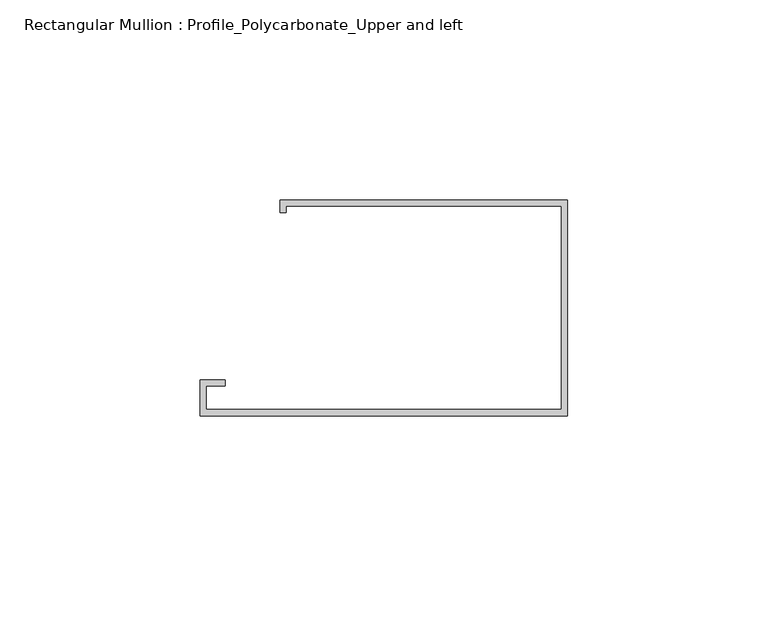
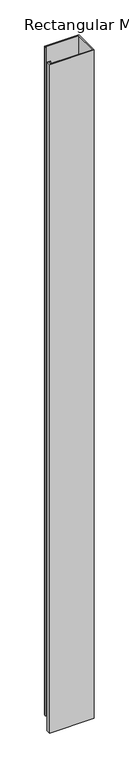
"""IFC4 building model written with IfcOpenShell, lengths in millimetres: member geometry, Rectangular Mullion : Profile_Polycarbonate_Upper and left."""

import ifcopenshell
import ifcopenshell.guid

model = None  # the IFC model being written
_history = None  # IfcOwnerHistory: only IFC2X3 demands one
_inside = {}  # id of a spatial element -> (the spatial element, [elements in it])
_under = {}  # id of a project, library or spatial element -> (it, [spatial elements below it])
_declared = {}  # id of a project -> (the project, [libraries it declares])
_typed = {}  # id of a type object -> (the type object, [elements of that type])
_made_of = {}  # id of a material, layer set ... -> (it, [elements and type objects made of it])


def new_model(schema):
    """Start an empty IFC model of exactly this schema.

    Asked for "IFC4X3", IfcOpenShell would pick the latest addendum, in which some entities
    have other attributes; the version numbers below select the first issue.
    IFC2X3 requires an IfcOwnerHistory on every rooted entity: one is made here for all.
    """
    global model, _history
    if schema == "IFC4X3":
        model = ifcopenshell.file(schema_version=(4, 3, 0, 0))
    else:
        model = ifcopenshell.file(schema=schema)
    _inside.clear()
    _under.clear()
    _declared.clear()
    _typed.clear()
    _made_of.clear()
    _history = None
    if model.schema == "IFC2X3":
        org = make("IfcOrganization", Name="unknown")
        user = make(
            "IfcPersonAndOrganization",
            ThePerson=make("IfcPerson", FamilyName="unknown"),
            TheOrganization=org,
        )
        app = make(
            "IfcApplication",
            ApplicationDeveloper=org,
            Version="unknown",
            ApplicationFullName="unknown",
            ApplicationIdentifier="unknown",
        )
        _history = make(
            "IfcOwnerHistory",
            OwningUser=user,
            OwningApplication=app,
            ChangeAction="ADDED",
            CreationDate=0,
        )
    return model


def make(cls, **values):
    """One entity of the class cls with the attributes given. An attribute that is None is left unset."""
    return model.create_entity(
        cls, **{name: value for name, value in values.items() if value is not None}
    )


def rooted(cls, **values):
    """An entity with a GlobalId (a new one), such as an element, a storey or a relation."""
    return make(cls, GlobalId=ifcopenshell.guid.new(), OwnerHistory=_history, **values)


def si_unit(unit_type, name, prefix=None):
    """IfcSIUnit, for example si_unit("LENGTHUNIT", "METRE", prefix="MILLI")."""
    return make("IfcSIUnit", UnitType=unit_type, Prefix=prefix, Name=name)


def assignment(units):
    """IfcUnitAssignment: the units of a project."""
    return None if units is None else make("IfcUnitAssignment", Units=units)


def point(xyz):
    """IfcCartesianPoint."""
    return None if xyz is None else make("IfcCartesianPoint", Coordinates=xyz)


def direction(xyz):
    """IfcDirection."""
    return None if xyz is None else make("IfcDirection", DirectionRatios=xyz)


def frame(location, z_axis=None, x_axis=None):
    """IfcAxis2Placement3D, a coordinate frame: its origin and axes. An axis left out is left unset."""
    return make(
        "IfcAxis2Placement3D",
        Location=point(location),
        Axis=direction(z_axis),
        RefDirection=direction(x_axis),
    )


def origin():
    """The frame at (0, 0, 0) with its axes left unset."""
    return frame((0.0, 0.0, 0.0))


def place(relative_to, where):
    """IfcLocalPlacement: puts the frame where relative to a parent placement (None: the world)."""
    return make(
        "IfcLocalPlacement", PlacementRelTo=relative_to, RelativePlacement=where
    )


def context(
    kind, dimensions, precision=None, world=None, true_north=None, identifier=None
):
    """IfcGeometricRepresentationContext, for example the 3D "Model" context."""
    return make(
        "IfcGeometricRepresentationContext",
        ContextIdentifier=identifier,
        ContextType=kind,
        CoordinateSpaceDimension=dimensions,
        Precision=precision,
        WorldCoordinateSystem=world,
        TrueNorth=true_north,
    )


def project(units=None, contexts=None):
    """IfcProject with its units and contexts."""
    return rooted(
        "IfcProject",
        Name="project",
        RepresentationContexts=contexts,
        UnitsInContext=assignment(units),
    )


def spatial(cls, under=None, at=None, **own):
    """A site, building, storey or space (cls), placed at a placement, below another one or the project."""
    s = rooted(cls, ObjectPlacement=at, **own)
    if under is not None:
        _under.setdefault(under.id(), (under, []))[1].append(s)
    return s


def polyline(points):
    """IfcPolyline through the points."""
    return make("IfcPolyline", Points=[point(p) for p in points])


def outline(outer, holes=None, kind="AREA"):
    """IfcArbitraryClosedProfileDef: a profile drawn as a closed curve; with holes, ...WithVoids."""
    if holes is None:
        return make("IfcArbitraryClosedProfileDef", ProfileType=kind, OuterCurve=outer)
    return make(
        "IfcArbitraryProfileDefWithVoids",
        ProfileType=kind,
        OuterCurve=outer,
        InnerCurves=holes,
    )


def extrude(swept, where, along, depth):
    """IfcExtrudedAreaSolid: the profile swept, set in the frame where, extruded along a direction by depth."""
    return make(
        "IfcExtrudedAreaSolid",
        SweptArea=swept,
        Position=where,
        ExtrudedDirection=direction(along),
        Depth=depth,
    )


def shape(context_of_items, identifier, shape_type, items):
    """IfcShapeRepresentation: the items that make up one representation, for example the "Body"."""
    return make(
        "IfcShapeRepresentation",
        ContextOfItems=context_of_items,
        RepresentationIdentifier=identifier,
        RepresentationType=shape_type,
        Items=items,
    )


def source(mapping_origin, context_of_items, identifier, shape_type, items):
    """IfcRepresentationMap: a shape defined once, which mapped items show again and again."""
    return make(
        "IfcRepresentationMap",
        MappingOrigin=mapping_origin,
        MappedRepresentation=shape(context_of_items, identifier, shape_type, items),
    )


def transform(
    local_origin,
    x_axis=None,
    y_axis=None,
    z_axis=None,
    scale=None,
    scale2=None,
    scale3=None,
    uniform=True,
):
    """IfcCartesianTransformationOperator3D, or its non-uniform kind. x_axis, y_axis, z_axis: its Axis1, 2, 3."""
    if uniform:
        return make(
            "IfcCartesianTransformationOperator3D",
            Axis1=direction(x_axis),
            Axis2=direction(y_axis),
            LocalOrigin=point(local_origin),
            Scale=scale,
            Axis3=direction(z_axis),
        )
    return make(
        "IfcCartesianTransformationOperator3DnonUniform",
        Axis1=direction(x_axis),
        Axis2=direction(y_axis),
        LocalOrigin=point(local_origin),
        Scale=scale,
        Axis3=direction(z_axis),
        Scale2=scale2,
        Scale3=scale3,
    )


def mapped(mapping_source, mapping_target):
    """IfcMappedItem: shows the shape of a source again, moved by a transform."""
    return make(
        "IfcMappedItem", MappingSource=mapping_source, MappingTarget=mapping_target
    )


def made_of(thing, what):
    """Note that an element or type object is made of a material, layer set ...; save() writes the relation."""
    if what is not None:
        _made_of.setdefault(what.id(), (what, []))[1].append(thing)
    return thing


def element(
    cls,
    number,
    at=None,
    inside=None,
    cuts=None,
    type_object=None,
    material=None,
    context=None,
    identifier="Body",
    shape_type=None,
    held_by="IfcProductDefinitionShape",
    body=None,
    shapes=None,
    **own,
):
    """One element of the class cls, such as IfcWall. Its Tag is "e" and its number.

    at: its placement. inside: the storey or other place that contains it. cuts: it is an
    opening in that element (IfcRelVoidsElement). A single representation is given by context,
    identifier, shape_type and body (its items); several are given by shapes. held_by: the class
    of the entity that holds the representations. save() writes the other relations.
    """
    e = rooted(cls, Tag="e%d" % number, ObjectPlacement=at, **own)
    if body is not None:
        shapes = [shape(context, identifier, shape_type, body)]
    if shapes is not None:
        e.Representation = make(held_by, Representations=shapes)
    if inside is not None:
        _inside.setdefault(inside.id(), (inside, []))[1].append(e)
    if cuts is not None:
        rooted(
            "IfcRelVoidsElement", RelatingBuildingElement=cuts, RelatedOpeningElement=e
        )
    if type_object is not None:
        _typed.setdefault(type_object.id(), (type_object, []))[1].append(e)
    return made_of(e, material)


def aggregate(whole, parts):
    """IfcRelAggregates: a whole, such as a stair, and the parts it consists of."""
    return rooted("IfcRelAggregates", RelatingObject=whole, RelatedObjects=parts)


def save(model, path):
    """Write the relations noted so far, then the file.

    IfcRelAggregates (storeys below a building ...), IfcRelContainedInSpatialStructure (elements
    in a storey), IfcRelDefinesByType, IfcRelAssociatesMaterial and IfcRelDeclares: one each for
    every whole, place, type object, material and project.
    """
    for whole, parts in _under.values():
        aggregate(whole, parts)
    for where, things in _inside.values():
        rooted(
            "IfcRelContainedInSpatialStructure",
            RelatedElements=things,
            RelatingStructure=where,
        )
    for kind, things in _typed.values():
        rooted("IfcRelDefinesByType", RelatedObjects=things, RelatingType=kind)
    for what, things in _made_of.values():
        rooted("IfcRelAssociatesMaterial", RelatedObjects=things, RelatingMaterial=what)
    for by, libraries in _declared.values():
        rooted("IfcRelDeclares", RelatingContext=by, RelatedDefinitions=libraries)
    model.write(path)


def rectangular_mullion_profile_polycarbonate_upper_and_left_cc2fb577(model_context):
    return source(origin(), model_context, "Body", "SweptSolid", [
        extrude(outline(polyline([(0.0, -28.984575), (-91.9988, -28.984575), (-91.9988, -19.992975), (-85.6488, -19.992975), (-85.6488, -21.580475), (-90.4113, -21.580475), (-90.4113, -27.397075), (-1.5875, -27.397075), (-1.5875, 23.428325), (-70.3961, 23.428325), (-70.3961, 21.840825), (-71.9836, 21.840825), (-71.9836, 25.015825), (0.0, 25.015825), (0.0, -28.984575)])), frame((0.0, 0.0, -1465.990511), z_axis=(0.0, 0.0, 1.0), x_axis=(1.0, 0.0, 0.0)), (0.0, 0.0, 1.0), 1465.990511),
    ])


if __name__ == "__main__":
    model = new_model("IFC4")
    model_context = context("Model", 3, world=origin())
    ifc_project = project(units=[si_unit("LENGTHUNIT", "METRE", prefix="MILLI")], contexts=[model_context])
    site = spatial("IfcSite", under=ifc_project)
    building = spatial("IfcBuilding", under=site)
    placement = place(None, origin())
    rectangular_mullion_profile_polycarbonate_upper_and_left_shape = rectangular_mullion_profile_polycarbonate_upper_and_left_cc2fb577(model_context)
    element("IfcMember", 1, ObjectType="Rectangular Mullion : Profile_Polycarbonate_Upper and left", at=placement, inside=building, context=model_context, shape_type="MappedRepresentation", body=[
        mapped(rectangular_mullion_profile_polycarbonate_upper_and_left_shape, transform((0.0, 0.0, 0.0), x_axis=(1.0, 0.0, 0.0), y_axis=(0.0, 1.0, 0.0), z_axis=(0.0, 0.0, 1.0))),
    ])
    save(model, "model.ifc")

# Revit data of these elements
# Type "Rectangular Mullion : Profile_Polycarbonate_Upper and left"
#   built-in parameter 1007322 = 0.177167 (stored number, unit not read)
#   built-in parameter 1007321 = 0.00520833 (stored number, unit not read)
#   built-in parameter 1007320 = 0 (stored number, unit not read)
